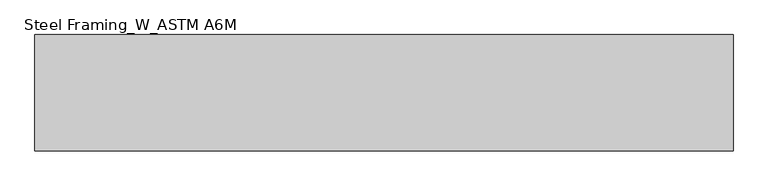
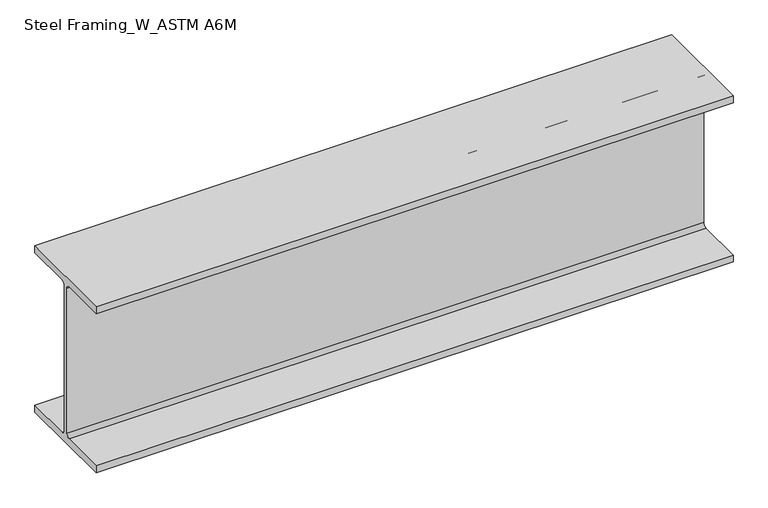
"""IFC4 building model written with IfcOpenShell, lengths in millimetres: beam geometry, Steel Framing_W_ASTM A6M : H_SB_AR_S02_W460x128_B1."""

from ifc_helpers import new_model, si_unit, point, frame, frame_2d, origin, place, context, project, spatial, polyline, circle_curve, trimmed, segment, composite_curve, outline, extrude, source, transform, mapped, element, save


def steel_framing_w_astm_a6m_954fd32e(model_context):
    return source(origin(), model_context, "Body", "SweptSolid", [
        extrude(outline(composite_curve([segment(polyline([(141.0, -213.9), (141.0, -233.5), (-141.0, -233.5), (-141.0, -213.9), (-16.2, -213.9)]), True, "CONTINUOUS"), segment(trimmed(circle_curve(frame_2d((-16.2, -203.8)), 10.1), [point((-16.2, -213.9))], [point((-6.1, -203.8))], True, "CARTESIAN"), True, "CONTINUOUS"), segment(polyline([(-6.1, -203.8), (-6.1, 203.8)]), True, "CONTINUOUS"), segment(trimmed(circle_curve(frame_2d((-16.2, 203.8)), 10.1), [point((-6.1, 203.8))], [point((-16.2, 213.9))], True, "CARTESIAN"), True, "CONTINUOUS"), segment(polyline([(-16.2, 213.9), (-141.0, 213.9), (-141.0, 233.5), (141.0, 233.5), (141.0, 213.9), (16.2, 213.9)]), True, "CONTINUOUS"), segment(trimmed(circle_curve(frame_2d((16.2, 203.8)), 10.1), [point((16.2, 213.9))], [point((6.1, 203.8))], True, "CARTESIAN"), True, "CONTINUOUS"), segment(polyline([(6.1, 203.8), (6.1, -203.8)]), True, "CONTINUOUS"), segment(trimmed(circle_curve(frame_2d((16.2, -203.8)), 10.1), [point((6.1, -203.8))], [point((16.2, -213.9))], True, "CARTESIAN"), True, "CONTINUOUS"), segment(polyline([(16.2, -213.9), (141.0, -213.9)]), True, "CONTINUOUS")], self_intersect=False)), frame((-846.3, 0.0, 0.0), z_axis=(1.0, 0.0, 0.0), x_axis=(0.0, 1.0, 0.0)), (0.0, 0.0, 1.0), 1692.6),
    ])


if __name__ == "__main__":
    model = new_model("IFC4")
    model_context = context("Model", 3, world=origin())
    ifc_project = project(units=[si_unit("LENGTHUNIT", "METRE", prefix="MILLI")], contexts=[model_context])
    site = spatial("IfcSite", under=ifc_project)
    building = spatial("IfcBuilding", under=site)
    placement = place(None, origin())
    steel_framing_w_astm_a6m_shape = steel_framing_w_astm_a6m_954fd32e(model_context)
    element("IfcBeam", 1, ObjectType="Steel Framing_W_ASTM A6M : H_SB_AR_S02_W460x128_B1", at=placement, inside=building, context=model_context, shape_type="MappedRepresentation", body=[
        mapped(steel_framing_w_astm_a6m_shape, transform((0.0, 0.0, 0.0), x_axis=(1.0, 0.0, 0.0), y_axis=(0.0, 1.0, 0.0), z_axis=(0.0, 0.0, 1.0))),
    ])
    save(model, "model.ifc")

# Revit data of these elements
# Type "Steel Framing_W_ASTM A6M : H_SB_AR_S02_W460x128_B1"
#   Section Name Key = "W18x86"
#   Width = 28.2 cm
#   Web Thickness = 1.22 cm
#   Web Fillet = 1.01 cm
#   Warping Constant = 3650000.0 cm⁶
#   Torsional Moment of Inertia = 171.00 cm⁴
#   Section Area = 163.0 cm²
#   Plastic Modulus weak axis = 793.0 cm³
#   Plastic Modulus strong axis = 3050.0 cm³
#   Perimeter = 2.02 m²/m
#   Nominal Weight = 128.00 kgf/m
#   Moment of Inertia weak axis = 7280.00 cm⁴
#   Moment of Inertia strong axis = 63700.00 cm⁴
#   Height = 46.7 cm
#   Flange Thickness = 1.96 cm
#   Elastic Modulus weak axis = 518.0 cm³
#   Elastic Modulus strong axis = 2720.0 cm³
#   Centroid Vertical = 23.35 cm
#   Centroid Horizontal = 14.1 cm
#   Length [instance default] = 1500 mm
#   Structural Material [instance default] = Steel, 45-345
#   Bolt Spacing = 0
#   Assembly Code = ""
# Element 1 (IfcBeam, "Steel Framing_W_ASTM A6M : H_SB_AR_S02_W460x128_B1")
#   Materials on its faces: "Steel, 45-345"
# Materials
#   "Steel, 45-345": class "Metal", colour RGB 189 187 185, transparency 0, Description = "Steel 345 MPa", Cost = 0
